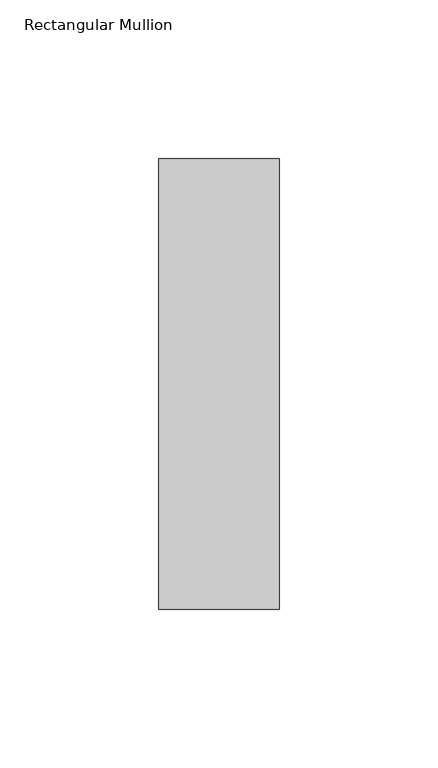
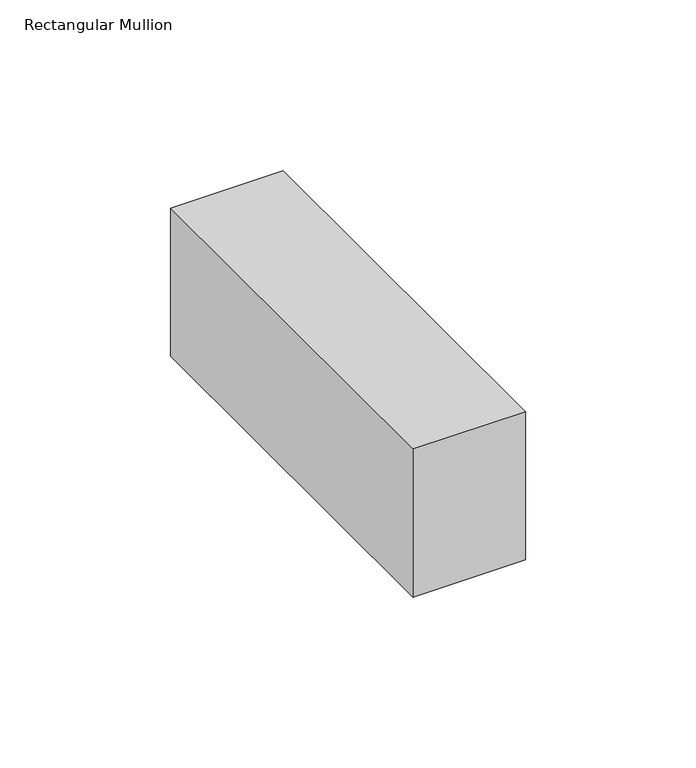
"""IFC4 building model written with IfcOpenShell, lengths in millimetres: member geometry, Rectangular Mullion : NLRS_21_CWM_hsb-regel 38x142_gen_rsf."""

from ifc_helpers import new_model, si_unit, frame, origin, place, context, project, spatial, polyline, outline, extrude, source, transform, mapped, element, save


def rectangular_mullion_03633001(model_context):
    return source(origin(), model_context, "Body", "SweptSolid", [
        extrude(outline(polyline([(0.0, -71.0), (-38.0, -71.0), (-38.0, 71.0), (0.0, 71.0), (0.0, -71.0)])), frame((0.0, 0.0, -52.9999997), z_axis=(0.0, 0.0, 1.0), x_axis=(1.0, 0.0, 0.0)), (0.0, 0.0, 1.0), 52.9999997),
    ])


if __name__ == "__main__":
    model = new_model("IFC4")
    model_context = context("Model", 3, world=origin())
    ifc_project = project(units=[si_unit("LENGTHUNIT", "METRE", prefix="MILLI")], contexts=[model_context])
    site = spatial("IfcSite", under=ifc_project)
    building = spatial("IfcBuilding", under=site)
    placement = place(None, origin())
    rectangular_mullion_shape = rectangular_mullion_03633001(model_context)
    element("IfcMember", 1, ObjectType="Rectangular Mullion : NLRS_21_CWM_hsb-regel 38x142_gen_rsf", at=placement, inside=building, context=model_context, shape_type="MappedRepresentation", body=[
        mapped(rectangular_mullion_shape, transform((0.0, 0.0, 0.0), x_axis=(1.0, 0.0, 0.0), y_axis=(0.0, 1.0, 0.0), z_axis=(0.0, 0.0, 1.0))),
    ])
    save(model, "model.ifc")

# Revit data of these elements
# Type "Rectangular Mullion : NLRS_21_CWM_hsb-regel 38x142_gen_rsf"
#   Export Type to IFC As = "IfcWall"
#   Type IfcGUID = "07M7mRoiH1CR8m_RSKIwpF"
#   Assembly Code = "21.10"
#   built-in parameter 1007322 = 0.465879 (stored number, unit not read)
#   built-in parameter 1007321 = 0.062336 (stored number, unit not read)
#   built-in parameter 1007320 = 0.062336 (stored number, unit not read)
# Element 1 (IfcMember, "Rectangular Mullion : NLRS_21_CWM_hsb-regel 38x142_gen_rsf")
#   Materials on its faces: "NLRS_i2_hout naaldhout vuren_gen_rsf"
# Materials
#   "NLRS_i2_hout naaldhout vuren_gen_rsf": class "I - Hout", colour RGB 234 199 147, transparency 0, Keynote = "i2", Manufacturer = "Revit Standards Foundation", URL = "www.revitstandards.org", Description = "hout vuren", Cost = 0
